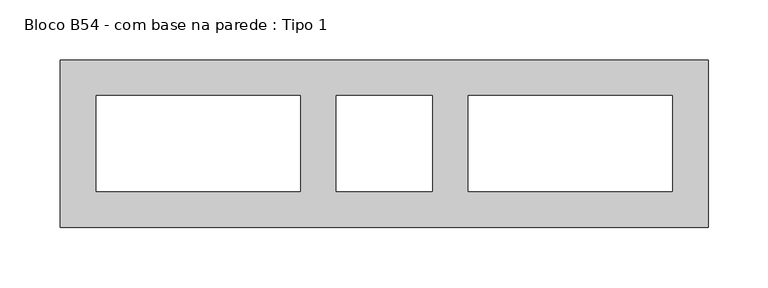
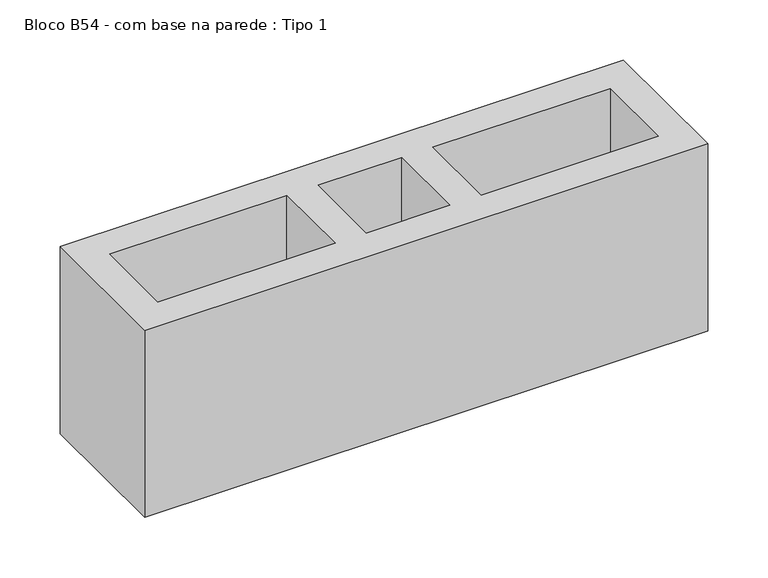
"""IFC4 building model written with IfcOpenShell, lengths in millimetres: proxy geometry, Bloco B54 - com base na parede : Tipo 1."""

from ifc_helpers import new_model, si_unit, origin, origin_with_axes, place, context, project, spatial, polyline, outline, extrude, source, transform, mapped, element, save


def bloco_b54_com_base_na_parede_tipo_1_a4c37ce6(model_context):
    return source(origin(), model_context, "Body", "SweptSolid", [
        extrude(outline(polyline([(320.0, 70.0), (320.0, -70.0), (-220.0, -70.0), (-220.0, 70.0), (320.0, 70.0)]), holes=[polyline([(120.0, 40.0), (120.0, -40.0), (290.0, -40.0), (290.0, 40.0), (120.0, 40.0)]), polyline([(-20.0, 40.0), (-190.0, 40.0), (-190.0, -40.0), (-20.0, -40.0), (-20.0, 40.0)]), polyline([(90.0, 40.0), (10.0, 40.0), (10.0, -40.0), (90.0, -40.0), (90.0, 40.0)])]), origin_with_axes(), (0.0, 0.0, 1.0), 190.0),
    ])


if __name__ == "__main__":
    model = new_model("IFC4")
    model_context = context("Model", 3, world=origin())
    ifc_project = project(units=[si_unit("LENGTHUNIT", "METRE", prefix="MILLI")], contexts=[model_context])
    site = spatial("IfcSite", under=ifc_project)
    building = spatial("IfcBuilding", under=site)
    placement = place(None, origin())
    bloco_b54_com_base_na_parede_tipo_1_shape = bloco_b54_com_base_na_parede_tipo_1_a4c37ce6(model_context)
    element("IfcBuildingElementProxy", 1, Name="Bloco B54 - com base na parede : Tipo 1", ObjectType="Bloco B54 - com base na parede : Tipo 1", at=placement, inside=building, context=model_context, shape_type="MappedRepresentation", body=[
        mapped(bloco_b54_com_base_na_parede_tipo_1_shape, transform((0.0, 0.0, 0.0), x_axis=(1.0, 0.0, 0.0), y_axis=(0.0, 1.0, 0.0), z_axis=(0.0, 0.0, 1.0))),
    ])
    save(model, "model.ifc")

# Revit data of these elements
# Type "Bloco B54 - com base na parede : Tipo 1"
#   SINAPI = ""
#   Assembly Code = ""
